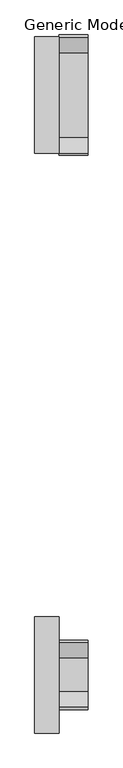
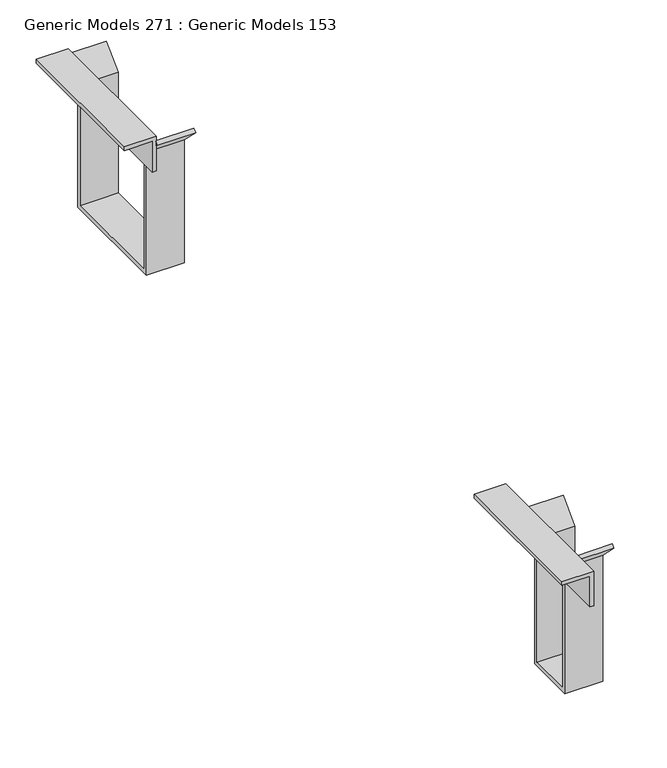
"""IFC4 building model written with IfcOpenShell, lengths in millimetres: proxy geometry, Generic Models 271 : Generic Models 153."""

from ifc_helpers import new_model, si_unit, frame, origin, place, context, project, spatial, polyline, outline, extrude, source, transform, mapped, element, save


def generic_models_271_generic_models_153_f80429a9(model_context):
    return source(origin(), model_context, "Body", "SweptSolid", [
        extrude(outline(polyline([(34845.3118167, 266326.9375), (34845.3118167, 266065.0), (34934.2118167, 266065.0), (34934.2118167, 266326.9375), (34975.0053266, 266367.7310099), (34980.6179867, 266362.1183498), (34942.1493167, 266323.6496798), (34942.1493167, 266057.0625), (34837.3743167, 266057.0625), (34837.3743167, 266323.6496798), (34798.9056467, 266362.1183498), (34804.5183068, 266367.7310099), (34845.3118167, 266326.9375)])), frame((32175.4585525, 0.0, 0.0), z_axis=(1.0, 0.0, 0.0), x_axis=(0.0, 1.0, 0.0)), (0.0, 0.0, 1.0), 76.2),
        extrude(outline(polyline([(266369.8, 32111.9585525), (266369.8, 32167.5210525), (266304.7125, 32167.5210525), (266304.7125, 32175.4585525), (266377.7375, 32175.4585525), (266377.7375, 32111.9585525), (266369.8, 32111.9585525)])), frame((0.0, 34737.3618167, 0.0), z_axis=(0.0, 1.0, 0.0), x_axis=(0.0, 0.0, 1.0)), (0.0, 0.0, 1.0), 304.8),
        extrude(outline(polyline([(36296.2957942, 266326.9375), (36296.2957942, 266071.35), (36518.5457942, 266071.35), (36518.5457942, 266326.9375), (36559.3393041, 266367.7310099), (36564.9519642, 266362.1183498), (36526.4832942, 266323.6496798), (36526.4832942, 266063.4125), (36288.3582942, 266063.4125), (36288.3582942, 266323.6496798), (36249.8896242, 266362.1183498), (36255.5022843, 266367.7310099), (36296.2957942, 266326.9375)])), frame((32175.4585525, 0.0, 0.0), z_axis=(1.0, 0.0, 0.0), x_axis=(0.0, 1.0, 0.0)), (0.0, 0.0, 1.0), 76.2),
        extrude(outline(polyline([(266369.8, 32111.9585525), (266369.8, 32167.5210525), (266304.7125, 32167.5210525), (266304.7125, 32175.4585525), (266377.7375, 32175.4585525), (266377.7375, 32111.9585525), (266369.8, 32111.9585525)])), frame((0.0, 36255.0207942, 0.0), z_axis=(0.0, 1.0, 0.0), x_axis=(0.0, 0.0, 1.0)), (0.0, 0.0, 1.0), 304.8),
    ])


if __name__ == "__main__":
    model = new_model("IFC4")
    model_context = context("Model", 3, world=origin())
    ifc_project = project(units=[si_unit("LENGTHUNIT", "METRE", prefix="MILLI")], contexts=[model_context])
    site = spatial("IfcSite", under=ifc_project)
    building = spatial("IfcBuilding", under=site)
    placement = place(None, origin())
    generic_models_271_generic_models_153_shape = generic_models_271_generic_models_153_f80429a9(model_context)
    element("IfcBuildingElementProxy", 1, Name="Generic Models 271 : Generic Models 153", ObjectType="Generic Models 271 : Generic Models 153", at=placement, inside=building, context=model_context, shape_type="MappedRepresentation", body=[
        mapped(generic_models_271_generic_models_153_shape, transform((0.0, 0.0, 0.0), x_axis=(1.0, 0.0, 0.0), y_axis=(0.0, 1.0, 0.0), z_axis=(0.0, 0.0, 1.0))),
    ])
    save(model, "model.ifc")

# Revit data of these elements
# Element 1 (IfcBuildingElementProxy, "Generic Models 271 : Generic Models 153")
#   Materials on its faces: "SIMPSON GLT HANGER (GALVANIZED)", "SIMPSON HGLT HANGER (GALVANIZED)"
# Materials
#   "SIMPSON GLT HANGER (GALVANIZED)": class "Metal", colour RGB 199 199 199, transparency 0, Description = "Carbon steel", Cost = 0
#   "SIMPSON HGLT HANGER (GALVANIZED)": class "Metal", colour RGB 199 199 199, transparency 0, Description = "Carbon steel", Cost = 0
